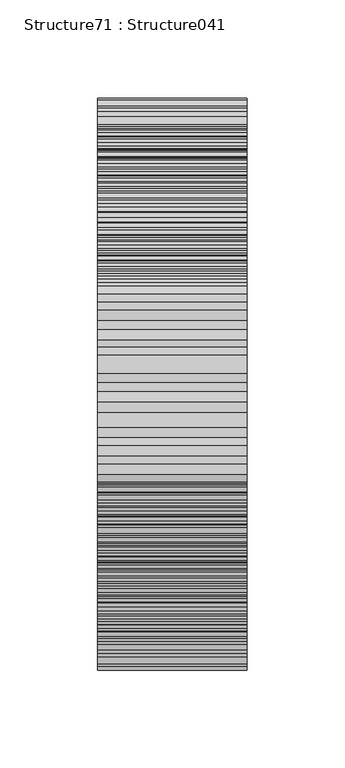
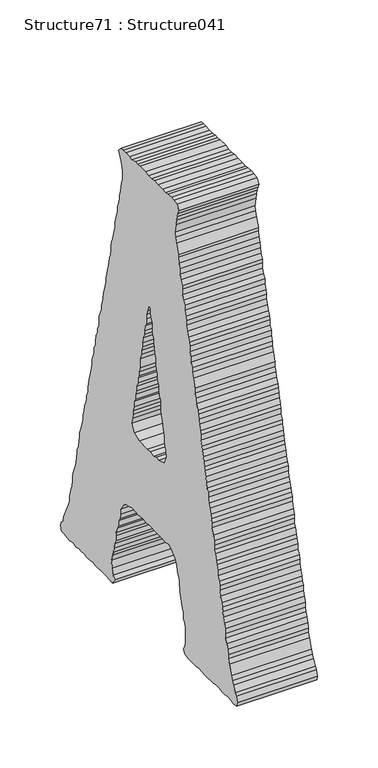
"""IFC4 building model written with IfcOpenShell, lengths in millimetres: proxy geometry, Structure71 : Structure041."""

from ifc_helpers import new_model, si_unit, frame, origin, place, context, project, spatial, polyline, outline, extrude, source, transform, mapped, element, save


def structure71_structure041_2c6c15dd(model_context):
    return source(origin(), model_context, "Body", "SweptSolid", [
        extrude(outline(polyline([(276960.0078056, 3818.8310229), (276960.0078056, 3814.7296538), (276961.1887945, 3811.2043377), (276963.507448, 3805.9476534), (276963.507448, 3801.8462843), (276964.1091747, 3795.960595), (276966.448688, 3791.8865042), (276966.448688, 3787.7867397), (276968.8106658, 3783.0868532), (276969.3899281, 3777.8285642), (276969.3899281, 3773.11905), (276971.731046, 3769.6274306), (276971.731046, 3763.759392), (276973.4912971, 3759.6596275), (276975.2515483, 3755.559863), (276975.2515483, 3750.8583719), (276976.4100727, 3746.1745313), (276978.7511907, 3737.400554), (276979.9321796, 3732.1149867), (276981.090704, 3727.4311462), (276982.2716929, 3723.3313817), (276982.2716929, 3718.6571688), (276984.0319441, 3713.3555556), (276984.6336708, 3709.2718371), (276986.373062, 3704.5879966), (276987.5540509, 3701.0723082), (276988.1333132, 3695.786741), (276989.8935643, 3690.512406), (276989.8935643, 3685.8285655), (276991.0745532, 3682.8857208), (276992.2346823, 3677.6274319), (276993.9949334, 3672.9435914), (276995.7551845, 3668.8261762), (276996.3344467, 3664.1423357), (276996.913709, 3660.0682449), (276997.5154357, 3654.1841602), (276999.8565536, 3650.1004418), (277000.4582803, 3645.9830266), (277001.0150781, 3641.2991861), (277001.5943403, 3636.0408972), (277002.7753292, 3631.915459), (277004.5355803, 3627.8397636), (277006.2958315, 3622.555801), (277007.478425, 3617.2718384), (277007.478425, 3613.772196), (277008.0576872, 3607.8961343), (277009.8179383, 3604.3964919), (277010.9764628, 3600.2967274), (277012.1574517, 3595.5872132), (277012.7367139, 3589.7544759), (277013.9177028, 3586.2115092), (277018.0190719, 3577.4535778), (277020.3585853, 3572.1423369), (277022.120441, 3568.6426945), (277023.2789654, 3563.366755), (277026.2202055, 3560.441561), (277027.4011944, 3556.3417965), (277025.6184788, 3551.6675836), (277020.9603119, 3551.6675836), (277016.2588208, 3551.0658569), (277012.1574517, 3550.4833855), (277006.8975581, 3551.6675836), (277001.5943403, 3550.4833855), (276996.913709, 3551.6675836), (276993.3932067, 3551.0658569), (276987.5540509, 3551.6675836), (276984.0319441, 3551.0658569), (276978.1943929, 3551.0658569), (276974.0705594, 3551.6675836), (276969.9707949, 3551.0658569), (276965.2676991, 3551.0658569), (276960.6095323, 3551.6675836), (276951.2274098, 3551.6675836), (276946.5467785, 3551.0658569), (276941.2435606, 3550.4833855), (276937.7439182, 3556.3417965), (276940.6642984, 3559.2669905), (276942.4245495, 3565.1254015), (276943.0038117, 3572.7440636), (276941.2435606, 3578.6104977), (276939.5041693, 3582.7102621), (276938.9249071, 3587.3860796), (276938.3456449, 3592.0955938), (276935.9836671, 3596.7698067), (276935.9836671, 3601.4536473), (276935.4044048, 3604.9709403), (276934.2234159, 3610.2292293), (276931.882298, 3613.772196), (276931.3030357, 3619.6145609), (276929.5427846, 3622.555801), (276928.3617957, 3627.8397636), (276928.3617957, 3633.0980525), (276923.6811644, 3639.5405396), (276920.1606621, 3643.0578326), (276913.1405175, 3644.8245022), (276909.6184106, 3645.9830266), (276903.758395, 3645.4262289), (276899.6570259, 3644.8245022), (276894.9763946, 3645.4262289), (276890.2749034, 3645.9830266), (276886.1959988, 3644.8245022), (276880.8927809, 3645.4262289), (276868.6127427, 3645.4262289), (276862.7511225, 3644.8245022), (276853.369, 3644.8245022), (276848.6883687, 3645.9830266), (276842.2474862, 3642.4833842), (276838.1252573, 3638.9580681), (276835.2273416, 3633.0980525), (276834.0463527, 3627.2396415), (276832.2861015, 3622.555801), (276831.1051126, 3619.6145609), (276829.9241237, 3609.0723094), (276828.7655993, 3604.3964919), (276827.6054702, 3600.2967274), (276825.8452191, 3596.1953583), (276824.6642302, 3592.0955938), (276824.0849679, 3586.2115092), (276822.3022524, 3582.7102621), (276821.1437279, 3578.6104977), (276821.1437279, 3573.9266571), (276821.1437279, 3563.9412034), (276822.3022524, 3559.2669905), (276824.0849679, 3555.7416744), (276821.7229901, 3551.6675836), (276816.4630966, 3550.4833855), (276802.979605, 3550.4833855), (276798.8798405, 3551.6675836), (276793.5974825, 3551.0658569), (276788.9168512, 3550.4833855), (276784.8170867, 3550.4833855), (276778.9554665, 3551.0658569), (276774.8765619, 3551.0658569), (276770.1750707, 3551.6675836), (276766.0737016, 3551.6675836), (276761.3722104, 3550.4833855), (276756.1123169, 3550.4833855), (276751.4316856, 3551.6675836), (276746.1284677, 3551.0658569), (276742.6288253, 3550.4833855), (276736.7896696, 3551.0658569), (276735.6086807, 3555.1848766), (276737.3689318, 3560.441561), (276738.5274562, 3563.366755), (276742.0495631, 3568.6426945), (276743.8098142, 3572.1423369), (276745.5700654, 3576.2693797), (276748.4904456, 3586.2115092), (276750.2506967, 3590.3289243), (276750.2506967, 3594.4286888), (276751.4316856, 3599.1125293), (276752.6126745, 3604.3964919), (276754.931328, 3608.4705827), (276755.5105902, 3612.5976255), (276755.5105902, 3617.2718384), (276756.6915791, 3622.555801), (276758.4518303, 3627.2396415), (276759.0535569, 3632.5155811), (276760.2120814, 3636.0408972), (276761.3722104, 3640.114988), (276763.1324616, 3645.4262289), (276764.3134505, 3650.6845178), (276764.3134505, 3655.3587307), (276765.4944394, 3659.4584952), (276767.8339527, 3663.5598643), (276767.8339527, 3668.8261762), (276769.573344, 3673.5276674), (276770.1750707, 3677.0449605), (276771.9353218, 3682.8857208), (276773.0938463, 3686.4030139), (276773.0938463, 3691.0868544), (276773.695573, 3695.2122926), (276774.8765619, 3699.8881101), (276777.1952154, 3705.7545441), (276777.1952154, 3710.4560353), (276778.3762043, 3714.5301261), (276779.5571932, 3718.0554422), (276780.7157176, 3723.3313817), (276782.4759688, 3727.4311462), (276783.6360978, 3732.7167134), (276783.6360978, 3737.9750024), (276785.396349, 3740.9162424), (276786.5773379, 3745.6000829), (276787.1566001, 3751.4424479), (276788.9168512, 3756.1423345), (276790.0978401, 3759.6596275), (276790.6771023, 3764.3611187), (276791.2579692, 3769.0176809), (276793.0182203, 3774.3032481), (276793.5974825, 3777.8285642), (276795.3577337, 3783.0868532), (276795.3577337, 3788.3611881), (276796.5387226, 3791.8865042), (276798.2781138, 3797.1463977), (276798.8798405, 3801.8462843), (276800.038365, 3806.5317294), (276800.6400917, 3810.0474179), (276802.979605, 3815.3313805), (276804.1605939, 3820.015221), (276805.3415828, 3824.1149855), (276805.3415828, 3829.374879), (276808.261963, 3837.6000817), (276809.4204875, 3842.8583706), (276810.0222141, 3846.9757858), (276811.7824653, 3851.6612309), (276811.7824653, 3856.9179152), (276813.5218566, 3861.0192843), (276814.1011188, 3866.3032469), (276814.7028455, 3869.8189354), (276816.4630966, 3873.9203044), (276818.2233477, 3878.5784713), (276819.4043366, 3883.8881076), (276819.4043366, 3888.5623205), (276820.5628611, 3892.6636896), (276822.3022524, 3897.3475301), (276822.3022524, 3902.6314927), (276824.6642302, 3906.1487857), (276825.8452191, 3910.8310217), (276826.4244813, 3916.0909152), (276826.4244813, 3919.6066036), (276828.7655993, 3924.2888396), (276829.9241237, 3928.9919353), (276830.5258504, 3934.2758979), (276831.6843748, 3938.9517154), (276832.8653637, 3944.235678), (276832.8653637, 3947.1496398), (276836.3650062, 3956.5349715), (276837.5459951, 3961.794865), (276838.726984, 3965.8930249), (276836.9667328, 3974.7055128), (276835.7857439, 3979.9621971), (276835.2273416, 3983.4794902), (276834.0463527, 3987.5792547), (276831.6843748, 3991.6806238), (276835.2273416, 3996.390138), (276840.4872351, 3996.9645864), (276844.5661397, 3997.5486624), (276849.8693576, 3997.5486624), (276853.9482622, 3996.390138), (276859.2306202, 3996.9645864), (276866.8300271, 3996.9645864), (276872.133245, 3997.5486624), (276877.3931385, 3996.390138), (276882.0737698, 3996.390138), (276886.775261, 3997.5486624), (276896.1365236, 3997.5486624), (276900.2587526, 3996.9645864), (276903.758395, 3997.5486624), (276909.0391484, 3996.390138), (276913.7197797, 3996.390138), (276918.9796732, 3997.5486624), (276923.1019022, 3997.5486624), (276927.2032713, 3996.9645864), (276931.3030357, 3992.2614906), (276928.9635224, 3987.5792547), (276927.2032713, 3984.0635662), (276926.0222823, 3979.3781211), (276924.8621533, 3974.7055128), (276924.8621533, 3966.5043792), (276926.6015446, 3962.3757319), (276927.7825335, 3957.1190475), (276928.3617957, 3952.435207), (276930.1220468, 3947.7337158), (276930.1220468, 3944.235678), (276931.3030357, 3938.3499888), (276933.0648915, 3934.8503464), (276933.0648915, 3929.5904528), (276934.8026782, 3924.8905662), (276936.5629293, 3919.6066036), (276937.7439182, 3915.5068392), (276937.7439182, 3910.8310217), (276938.9249071, 3906.1487857), (276940.105896, 3902.6314927), (276941.2435606, 3896.763454), (276943.0038117, 3893.822214), (276944.1848006, 3888.5623205), (276944.1848006, 3884.4609514), (276944.7865273, 3878.5784713), (276946.5467785, 3875.0772243), (276947.1260407, 3870.4030114), (276948.2861697, 3866.3032469), (276949.4671586, 3861.0192843), (276950.6256831, 3856.9179152), (276952.3859342, 3851.6612309), (276952.3859342, 3846.9757858), (276954.1461853, 3841.6741725), (276954.747912, 3838.1761347), (276956.4873033, 3833.4730389), (276957.0665655, 3828.2163546), (276957.6682922, 3824.1149855), (276960.0078056, 3818.8310229)]), holes=[polyline([(276897.3175125, 3720.4158154), (276905.5186461, 3723.9154578), (276909.0391484, 3730.9323932), (276907.8581595, 3736.7988273), (276906.699635, 3741.5003184), (276906.699635, 3744.9999608), (276904.9169194, 3750.3015741), (276904.9169194, 3755.559863), (276903.1791327, 3759.0595054), (276902.5982659, 3764.3611187), (276901.417277, 3768.4432325), (276901.417277, 3773.11905), (276899.0777637, 3777.8285642), (276899.0777637, 3783.0868532), (276897.3175125, 3786.0280932), (276896.7157858, 3790.7039107), (276895.5781213, 3795.4037973), (276894.9763946, 3804.7730829), (276893.2161434, 3810.0474179), (276892.6368812, 3814.7296538), (276891.4558923, 3818.8310229), (276890.8766301, 3822.932392), (276890.2749034, 3828.790803), (276887.9562499, 3833.4730389), (276887.9562499, 3836.9919366), (276887.3545232, 3842.2758992), (276885.0150099, 3845.8012153), (276885.0150099, 3851.0595042), (276884.4357476, 3855.7353217), (276882.653032, 3860.4432313), (276881.4945076, 3865.1190488), (276879.7551163, 3864.5446004), (276879.7551163, 3860.4432313), (276878.5741274, 3856.3161885), (276876.8138763, 3851.6612309), (276876.8138763, 3846.3772683), (276876.2121496, 3842.2758992), (276873.8726362, 3837.6000817), (276873.8726362, 3832.8921721), (276873.293374, 3828.790803), (276872.133245, 3824.1149855), (276870.9522561, 3819.4150989), (276870.3729938, 3813.5743386), (276869.7712671, 3810.0474179), (276868.011016, 3805.9476534), (276868.011016, 3800.6717138), (276865.6715027, 3795.4037973), (276865.6715027, 3790.7039107), (276864.5113736, 3786.0280932), (276862.7511225, 3782.5027771), (276862.1718603, 3777.2444882), (276862.1718603, 3772.5606477), (276861.5701336, 3767.8607611), (276859.8098824, 3763.759392), (276859.2306202, 3759.6596275), (276858.6288935, 3754.9854146), (276856.31024, 3750.8583719), (276856.8895023, 3744.9999608), (276855.7085133, 3740.9162424), (276854.5499889, 3736.7988273), (276853.369, 3730.9323932), (276856.31024, 3723.3313817), (276865.0906358, 3720.4158154), (276869.1920049, 3720.9726131), (276873.293374, 3719.8140887), (276878.5741274, 3720.9726131), (276883.8340209, 3720.4158154), (276897.3175125, 3720.4158154)])]), frame((-59031.6926606, 0.0, 0.0), z_axis=(1.0, 0.0, 0.0), x_axis=(0.0, 1.0, 0.0)), (0.0, 0.0, 1.0), 76.2),
    ])


if __name__ == "__main__":
    model = new_model("IFC4")
    model_context = context("Model", 3, world=origin())
    ifc_project = project(units=[si_unit("LENGTHUNIT", "METRE", prefix="MILLI")], contexts=[model_context])
    site = spatial("IfcSite", under=ifc_project)
    building = spatial("IfcBuilding", under=site)
    placement = place(None, origin())
    structure71_structure041_shape = structure71_structure041_2c6c15dd(model_context)
    element("IfcBuildingElementProxy", 1, Name="Structure71 : Structure041", ObjectType="Structure71 : Structure041", at=placement, inside=building, context=model_context, shape_type="MappedRepresentation", body=[
        mapped(structure71_structure041_shape, transform((0.0, 0.0, 0.0), x_axis=(1.0, 0.0, 0.0), y_axis=(0.0, 1.0, 0.0), z_axis=(0.0, 0.0, 1.0))),
    ])
    save(model, "model.ifc")

# Revit data of these elements
# Type "Structure71 : Structure041"
#   NameOverride = "Structure041"
# Element 1 (IfcBuildingElementProxy, "Structure71 : Structure041")
#   Materials on its faces: "BRUSHED ALUM. LETTERING"
# Materials
#   "BRUSHED ALUM. LETTERING": class "Unassigned", colour RGB 169 181 186, transparency 0, Cost = 0
